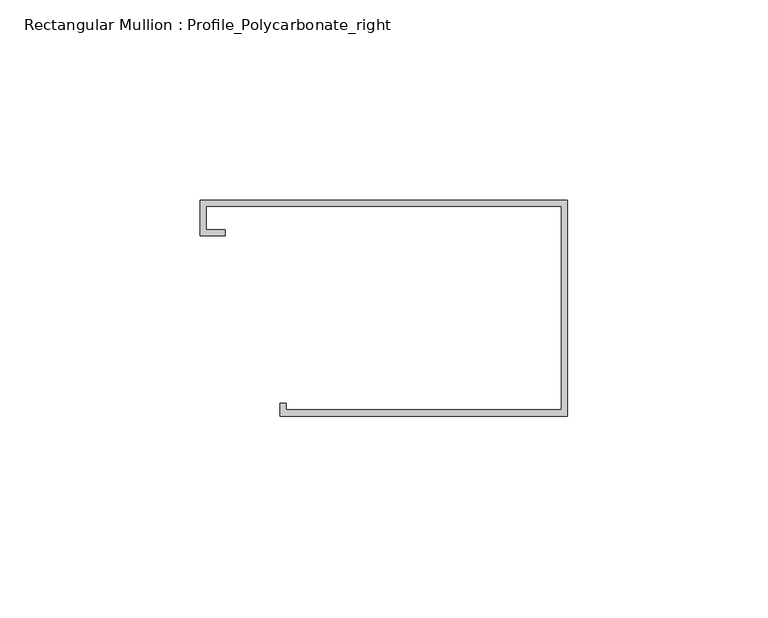
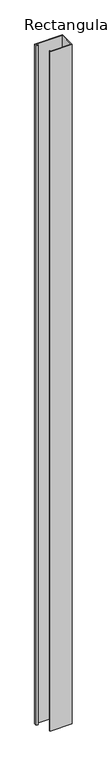
"""IFC4 building model written with IfcOpenShell, lengths in millimetres: member geometry, Rectangular Mullion : Profile_Polycarbonate_right."""

from ifc_helpers import new_model, si_unit, frame, origin, place, context, project, spatial, polyline, outline, extrude, source, transform, mapped, element, save


def rectangular_mullion_profile_polycarbonate_right_f43dabe3(model_context):
    return source(origin(), model_context, "Body", "SweptSolid", [
        extrude(outline(polyline([(0.0, 28.984575), (0.0, -25.015825), (-71.9836, -25.015825), (-71.9836, -21.840825), (-70.3961, -21.840825), (-70.3961, -23.428325), (-1.5875, -23.428325), (-1.5875, 27.397075), (-90.4113, 27.397075), (-90.4113, 21.580475), (-85.6488, 21.580475), (-85.6488, 19.992975), (-91.9988, 19.992975), (-91.9988, 28.984575), (0.0, 28.984575)])), frame((0.0, 0.0, -2369.6313366), z_axis=(0.0, 0.0, 1.0), x_axis=(1.0, 0.0, 0.0)), (0.0, 0.0, 1.0), 2369.6313366),
    ])


if __name__ == "__main__":
    model = new_model("IFC4")
    model_context = context("Model", 3, world=origin())
    ifc_project = project(units=[si_unit("LENGTHUNIT", "METRE", prefix="MILLI")], contexts=[model_context])
    site = spatial("IfcSite", under=ifc_project)
    building = spatial("IfcBuilding", under=site)
    placement = place(None, origin())
    rectangular_mullion_profile_polycarbonate_right_shape = rectangular_mullion_profile_polycarbonate_right_f43dabe3(model_context)
    element("IfcMember", 1, ObjectType="Rectangular Mullion : Profile_Polycarbonate_right", at=placement, inside=building, context=model_context, shape_type="MappedRepresentation", body=[
        mapped(rectangular_mullion_profile_polycarbonate_right_shape, transform((0.0, 0.0, 0.0), x_axis=(1.0, 0.0, 0.0), y_axis=(0.0, 1.0, 0.0), z_axis=(0.0, 0.0, 1.0))),
    ])
    save(model, "model.ifc")

# Revit data of these elements
# Type "Rectangular Mullion : Profile_Polycarbonate_right"
#   built-in parameter 1007322 = 0.177167 (stored number, unit not read)
#   built-in parameter 1007321 = 0 (stored number, unit not read)
#   built-in parameter 1007320 = 0.00520833 (stored number, unit not read)
